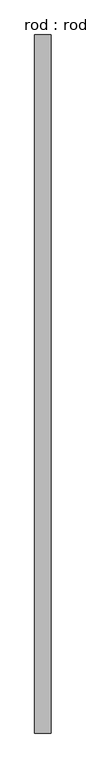
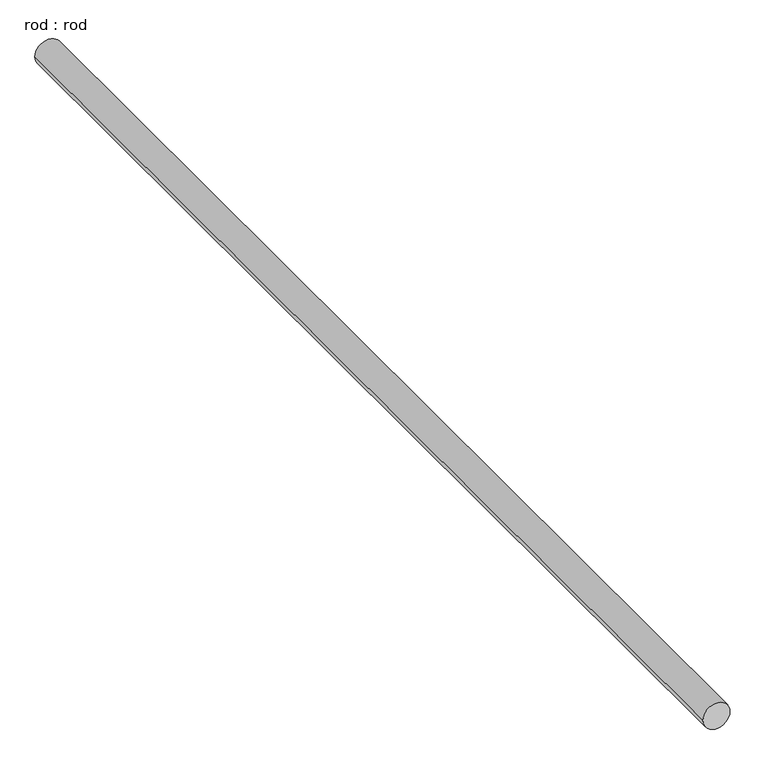
"""IFC4 building model written with IfcOpenShell, lengths in millimetres: proxy geometry, rod : rod."""

from ifc_helpers import new_model, si_unit, point, frame, frame_2d, origin, place, context, project, spatial, circle_curve, trimmed, segment, composite_curve, outline, extrude, source, transform, mapped, element, save


def rod_rod_d8a81dad(model_context):
    return source(origin(), model_context, "Body", "SweptSolid", [
        extrude(outline(composite_curve([segment(trimmed(circle_curve(frame_2d((0.0108462, 0.0)), 200.0), [point((0.0108462, 200.0))], [point((0.0108462, -200.0))], False, "CARTESIAN"), True, "CONTINUOUS"), segment(trimmed(circle_curve(frame_2d((0.0108462, 0.0)), 200.0), [point((0.0108462, -200.0))], [point((0.0108462, 200.0))], False, "CARTESIAN"), True, "CONTINUOUS")], self_intersect=False)), frame((0.0, -4465.3070989, 0.0), z_axis=(0.0, 1.0, 0.0), x_axis=(0.0, 0.0, 1.0)), (0.0, 0.0, 1.0), 17116.0714286),
    ])


if __name__ == "__main__":
    model = new_model("IFC4")
    model_context = context("Model", 3, world=origin())
    ifc_project = project(units=[si_unit("LENGTHUNIT", "METRE", prefix="MILLI")], contexts=[model_context])
    site = spatial("IfcSite", under=ifc_project)
    building = spatial("IfcBuilding", under=site)
    placement = place(None, origin())
    rod_rod_shape = rod_rod_d8a81dad(model_context)
    element("IfcBuildingElementProxy", 1, Name="rod : rod", ObjectType="rod : rod", at=placement, inside=building, context=model_context, shape_type="MappedRepresentation", body=[
        mapped(rod_rod_shape, transform((0.0, 0.0, 0.0), x_axis=(1.0, 0.0, 0.0), y_axis=(0.0, 1.0, 0.0), z_axis=(0.0, 0.0, 1.0))),
    ])
    save(model, "model.ifc")

# Revit data of these elements
# Type "rod : rod"
#   Default Elevation = 0
